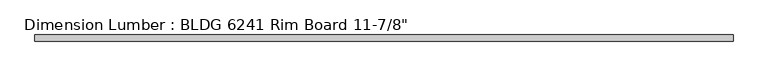
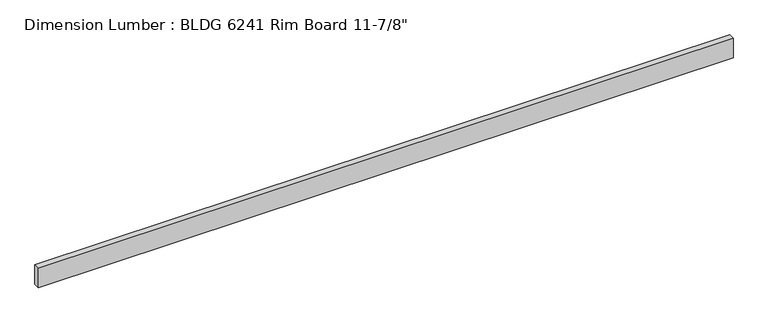
"""IFC4 building model written with IfcOpenShell, lengths in millimetres: beam geometry."""

import ifcopenshell
import ifcopenshell.guid

model = None  # the IFC model being written
_history = None  # IfcOwnerHistory: only IFC2X3 demands one
_inside = {}  # id of a spatial element -> (the spatial element, [elements in it])
_under = {}  # id of a project, library or spatial element -> (it, [spatial elements below it])
_declared = {}  # id of a project -> (the project, [libraries it declares])
_typed = {}  # id of a type object -> (the type object, [elements of that type])
_made_of = {}  # id of a material, layer set ... -> (it, [elements and type objects made of it])


def new_model(schema):
    """Start an empty IFC model of exactly this schema.

    Asked for "IFC4X3", IfcOpenShell would pick the latest addendum, in which some entities
    have other attributes; the version numbers below select the first issue.
    IFC2X3 requires an IfcOwnerHistory on every rooted entity: one is made here for all.
    """
    global model, _history
    if schema == "IFC4X3":
        model = ifcopenshell.file(schema_version=(4, 3, 0, 0))
    else:
        model = ifcopenshell.file(schema=schema)
    _inside.clear()
    _under.clear()
    _declared.clear()
    _typed.clear()
    _made_of.clear()
    _history = None
    if model.schema == "IFC2X3":
        org = make("IfcOrganization", Name="unknown")
        user = make(
            "IfcPersonAndOrganization",
            ThePerson=make("IfcPerson", FamilyName="unknown"),
            TheOrganization=org,
        )
        app = make(
            "IfcApplication",
            ApplicationDeveloper=org,
            Version="unknown",
            ApplicationFullName="unknown",
            ApplicationIdentifier="unknown",
        )
        _history = make(
            "IfcOwnerHistory",
            OwningUser=user,
            OwningApplication=app,
            ChangeAction="ADDED",
            CreationDate=0,
        )
    return model


def make(cls, **values):
    """One entity of the class cls with the attributes given. An attribute that is None is left unset."""
    return model.create_entity(
        cls, **{name: value for name, value in values.items() if value is not None}
    )


def rooted(cls, **values):
    """An entity with a GlobalId (a new one), such as an element, a storey or a relation."""
    return make(cls, GlobalId=ifcopenshell.guid.new(), OwnerHistory=_history, **values)


def si_unit(unit_type, name, prefix=None):
    """IfcSIUnit, for example si_unit("LENGTHUNIT", "METRE", prefix="MILLI")."""
    return make("IfcSIUnit", UnitType=unit_type, Prefix=prefix, Name=name)


def assignment(units):
    """IfcUnitAssignment: the units of a project."""
    return None if units is None else make("IfcUnitAssignment", Units=units)


def point(xyz):
    """IfcCartesianPoint."""
    return None if xyz is None else make("IfcCartesianPoint", Coordinates=xyz)


def direction(xyz):
    """IfcDirection."""
    return None if xyz is None else make("IfcDirection", DirectionRatios=xyz)


def frame(location, z_axis=None, x_axis=None):
    """IfcAxis2Placement3D, a coordinate frame: its origin and axes. An axis left out is left unset."""
    return make(
        "IfcAxis2Placement3D",
        Location=point(location),
        Axis=direction(z_axis),
        RefDirection=direction(x_axis),
    )


def origin():
    """The frame at (0, 0, 0) with its axes left unset."""
    return frame((0.0, 0.0, 0.0))


def place(relative_to, where):
    """IfcLocalPlacement: puts the frame where relative to a parent placement (None: the world)."""
    return make(
        "IfcLocalPlacement", PlacementRelTo=relative_to, RelativePlacement=where
    )


def context(
    kind, dimensions, precision=None, world=None, true_north=None, identifier=None
):
    """IfcGeometricRepresentationContext, for example the 3D "Model" context."""
    return make(
        "IfcGeometricRepresentationContext",
        ContextIdentifier=identifier,
        ContextType=kind,
        CoordinateSpaceDimension=dimensions,
        Precision=precision,
        WorldCoordinateSystem=world,
        TrueNorth=true_north,
    )


def project(units=None, contexts=None):
    """IfcProject with its units and contexts."""
    return rooted(
        "IfcProject",
        Name="project",
        RepresentationContexts=contexts,
        UnitsInContext=assignment(units),
    )


def spatial(cls, under=None, at=None, **own):
    """A site, building, storey or space (cls), placed at a placement, below another one or the project."""
    s = rooted(cls, ObjectPlacement=at, **own)
    if under is not None:
        _under.setdefault(under.id(), (under, []))[1].append(s)
    return s


def polyline(points):
    """IfcPolyline through the points."""
    return make("IfcPolyline", Points=[point(p) for p in points])


def outline(outer, holes=None, kind="AREA"):
    """IfcArbitraryClosedProfileDef: a profile drawn as a closed curve; with holes, ...WithVoids."""
    if holes is None:
        return make("IfcArbitraryClosedProfileDef", ProfileType=kind, OuterCurve=outer)
    return make(
        "IfcArbitraryProfileDefWithVoids",
        ProfileType=kind,
        OuterCurve=outer,
        InnerCurves=holes,
    )


def extrude(swept, where, along, depth):
    """IfcExtrudedAreaSolid: the profile swept, set in the frame where, extruded along a direction by depth."""
    return make(
        "IfcExtrudedAreaSolid",
        SweptArea=swept,
        Position=where,
        ExtrudedDirection=direction(along),
        Depth=depth,
    )


def shape(context_of_items, identifier, shape_type, items):
    """IfcShapeRepresentation: the items that make up one representation, for example the "Body"."""
    return make(
        "IfcShapeRepresentation",
        ContextOfItems=context_of_items,
        RepresentationIdentifier=identifier,
        RepresentationType=shape_type,
        Items=items,
    )


def source(mapping_origin, context_of_items, identifier, shape_type, items):
    """IfcRepresentationMap: a shape defined once, which mapped items show again and again."""
    return make(
        "IfcRepresentationMap",
        MappingOrigin=mapping_origin,
        MappedRepresentation=shape(context_of_items, identifier, shape_type, items),
    )


def transform(
    local_origin,
    x_axis=None,
    y_axis=None,
    z_axis=None,
    scale=None,
    scale2=None,
    scale3=None,
    uniform=True,
):
    """IfcCartesianTransformationOperator3D, or its non-uniform kind. x_axis, y_axis, z_axis: its Axis1, 2, 3."""
    if uniform:
        return make(
            "IfcCartesianTransformationOperator3D",
            Axis1=direction(x_axis),
            Axis2=direction(y_axis),
            LocalOrigin=point(local_origin),
            Scale=scale,
            Axis3=direction(z_axis),
        )
    return make(
        "IfcCartesianTransformationOperator3DnonUniform",
        Axis1=direction(x_axis),
        Axis2=direction(y_axis),
        LocalOrigin=point(local_origin),
        Scale=scale,
        Axis3=direction(z_axis),
        Scale2=scale2,
        Scale3=scale3,
    )


def mapped(mapping_source, mapping_target):
    """IfcMappedItem: shows the shape of a source again, moved by a transform."""
    return make(
        "IfcMappedItem", MappingSource=mapping_source, MappingTarget=mapping_target
    )


def made_of(thing, what):
    """Note that an element or type object is made of a material, layer set ...; save() writes the relation."""
    if what is not None:
        _made_of.setdefault(what.id(), (what, []))[1].append(thing)
    return thing


def element(
    cls,
    number,
    at=None,
    inside=None,
    cuts=None,
    type_object=None,
    material=None,
    context=None,
    identifier="Body",
    shape_type=None,
    held_by="IfcProductDefinitionShape",
    body=None,
    shapes=None,
    **own,
):
    """One element of the class cls, such as IfcWall. Its Tag is "e" and its number.

    at: its placement. inside: the storey or other place that contains it. cuts: it is an
    opening in that element (IfcRelVoidsElement). A single representation is given by context,
    identifier, shape_type and body (its items); several are given by shapes. held_by: the class
    of the entity that holds the representations. save() writes the other relations.
    """
    e = rooted(cls, Tag="e%d" % number, ObjectPlacement=at, **own)
    if body is not None:
        shapes = [shape(context, identifier, shape_type, body)]
    if shapes is not None:
        e.Representation = make(held_by, Representations=shapes)
    if inside is not None:
        _inside.setdefault(inside.id(), (inside, []))[1].append(e)
    if cuts is not None:
        rooted(
            "IfcRelVoidsElement", RelatingBuildingElement=cuts, RelatedOpeningElement=e
        )
    if type_object is not None:
        _typed.setdefault(type_object.id(), (type_object, []))[1].append(e)
    return made_of(e, material)


def aggregate(whole, parts):
    """IfcRelAggregates: a whole, such as a stair, and the parts it consists of."""
    return rooted("IfcRelAggregates", RelatingObject=whole, RelatedObjects=parts)


def save(model, path):
    """Write the relations noted so far, then the file.

    IfcRelAggregates (storeys below a building ...), IfcRelContainedInSpatialStructure (elements
    in a storey), IfcRelDefinesByType, IfcRelAssociatesMaterial and IfcRelDeclares: one each for
    every whole, place, type object, material and project.
    """
    for whole, parts in _under.values():
        aggregate(whole, parts)
    for where, things in _inside.values():
        rooted(
            "IfcRelContainedInSpatialStructure",
            RelatedElements=things,
            RelatingStructure=where,
        )
    for kind, things in _typed.values():
        rooted("IfcRelDefinesByType", RelatedObjects=things, RelatingType=kind)
    for what, things in _made_of.values():
        rooted("IfcRelAssociatesMaterial", RelatedObjects=things, RelatingMaterial=what)
    for by, libraries in _declared.values():
        rooted("IfcRelDeclares", RelatingContext=by, RelatedDefinitions=libraries)
    model.write(path)


def beam_ce0f0212(model_context):
    return source(origin(), model_context, "Body", "SweptSolid", [
        extrude(outline(polyline([(5041.9, 44.45), (5041.9, -44.45), (-5130.8, -44.45), (-5130.8, 44.45), (5041.9, 44.45)])), frame((0.0, 0.0, -150.8125), z_axis=(0.0, 0.0, 1.0), x_axis=(1.0, 0.0, 0.0)), (0.0, 0.0, 1.0), 301.625),
    ])


if __name__ == "__main__":
    model = new_model("IFC4")
    model_context = context("Model", 3, world=origin())
    ifc_project = project(units=[si_unit("LENGTHUNIT", "METRE", prefix="MILLI")], contexts=[model_context])
    site = spatial("IfcSite", under=ifc_project)
    building = spatial("IfcBuilding", under=site)
    placement = place(None, origin())
    beam_shape = beam_ce0f0212(model_context)
    element("IfcBeam", 1, ObjectType="Dimension Lumber : BLDG 6241 Rim Board 11-7/8\"", at=placement, inside=building, context=model_context, shape_type="MappedRepresentation", body=[
        mapped(beam_shape, transform((0.0, 0.0, 0.0), x_axis=(1.0, 0.0, 0.0), y_axis=(0.0, 1.0, 0.0), z_axis=(0.0, 0.0, 1.0))),
    ])
    save(model, "model.ifc")

# Revit data of these elements
# Type "Dimension Lumber : BLDG 6241 Rim Board 11-7/8\""
#   Assembly Code = "B10"
#   A = 0.273472 SF
#   Length [instance default] = 5' - 0"
#   b = 0' - 3 1/2"
#   d = 0' - 11 7/8"
#   Structural Material [instance default] = Softwood, Lumber
# Element 1 (IfcBeam, "Dimension Lumber : BLDG 6241 Rim Board 11-7/8\"")
#   Materials on its faces: "Softwood, Lumber"
# Materials
#   "Softwood, Lumber": class "Wood", colour RGB 223 192 134, transparency 0, Description = "Pinus Echinata", Cost = 0
